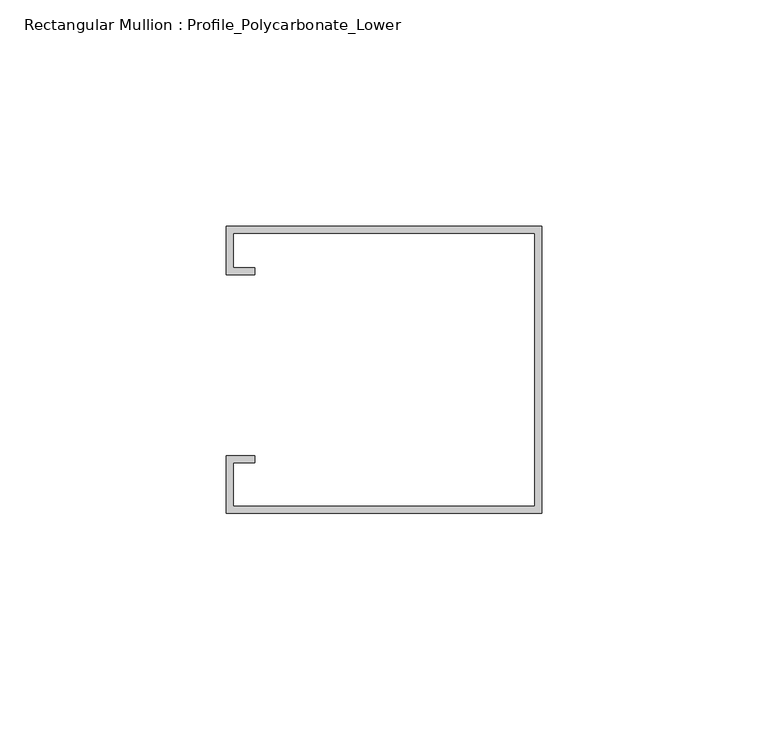
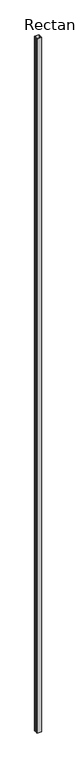
"""IFC4 building model written with IfcOpenShell, lengths in millimetres: member geometry, Rectangular Mullion : Profile_Polycarbonate_Lower."""

from ifc_helpers import new_model, si_unit, frame, origin, place, context, project, spatial, polyline, outline, extrude, source, transform, mapped, element, save


def rectangular_mullion_profile_polycarbonate_lower_fbcf21d4(model_context):
    return source(origin(), model_context, "Body", "SweptSolid", [
        extrude(outline(polyline([(0.0, -32.7), (-69.85, -32.7), (-69.85, -20.0), (-63.5, -20.0), (-63.5, -21.5875), (-68.2625, -21.5875), (-68.2625, -31.1125), (-1.5875, -31.1125), (-1.5875, 29.2125), (-68.2625, 29.2125), (-68.2625, 21.5875), (-63.5, 21.5875), (-63.5, 20.0), (-69.85, 20.0), (-69.85, 30.8), (0.0, 30.8), (0.0, -32.7)])), frame((0.0, 0.0, -11717.3375), z_axis=(0.0, 0.0, 1.0), x_axis=(1.0, 0.0, 0.0)), (0.0, 0.0, 1.0), 11717.3375),
    ])


if __name__ == "__main__":
    model = new_model("IFC4")
    model_context = context("Model", 3, world=origin())
    ifc_project = project(units=[si_unit("LENGTHUNIT", "METRE", prefix="MILLI")], contexts=[model_context])
    site = spatial("IfcSite", under=ifc_project)
    building = spatial("IfcBuilding", under=site)
    placement = place(None, origin())
    rectangular_mullion_profile_polycarbonate_lower_shape = rectangular_mullion_profile_polycarbonate_lower_fbcf21d4(model_context)
    element("IfcMember", 1, ObjectType="Rectangular Mullion : Profile_Polycarbonate_Lower", at=placement, inside=building, context=model_context, shape_type="MappedRepresentation", body=[
        mapped(rectangular_mullion_profile_polycarbonate_lower_shape, transform((0.0, 0.0, 0.0), x_axis=(1.0, 0.0, 0.0), y_axis=(0.0, 1.0, 0.0), z_axis=(0.0, 0.0, 1.0))),
    ])
    save(model, "model.ifc")

# Revit data of these elements
# Type "Rectangular Mullion : Profile_Polycarbonate_Lower"
#   built-in parameter 1007322 = 0.208333 (stored number, unit not read)
#   built-in parameter 1007321 = 0 (stored number, unit not read)
#   built-in parameter 1007320 = 0.00520833 (stored number, unit not read)
